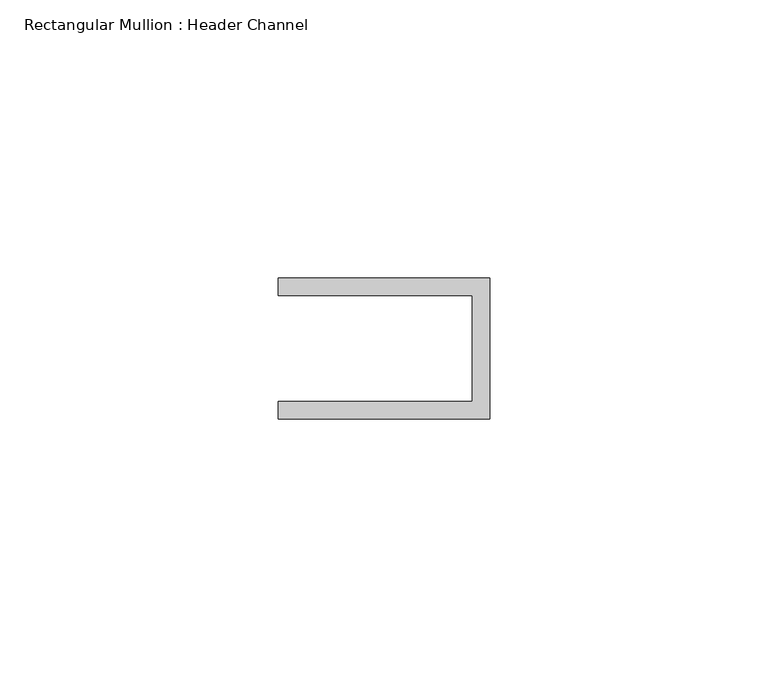
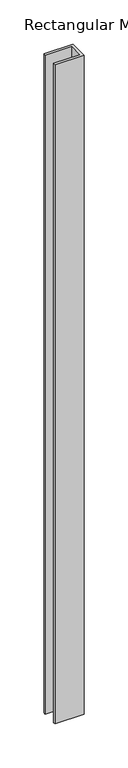
"""IFC4 building model written with IfcOpenShell, lengths in millimetres: member geometry, Rectangular Mullion : Header Channel."""

from ifc_helpers import new_model, si_unit, frame, origin, place, context, project, spatial, polyline, outline, extrude, source, transform, mapped, element, save


def rectangular_mullion_header_channel_2c3a6b86(model_context):
    return source(origin(), model_context, "Body", "SweptSolid", [
        extrude(outline(polyline([(0.0, -12.7), (-38.1, -12.7), (-38.1, -9.525), (-3.175, -9.525), (-3.175, 9.525), (-38.1, 9.525), (-38.1, 12.7), (0.0, 12.7), (0.0, -12.7)])), frame((0.0, 0.0, -914.4000002), z_axis=(0.0, 0.0, 1.0), x_axis=(1.0, 0.0, 0.0)), (0.0, 0.0, 1.0), 914.4000002),
    ])


if __name__ == "__main__":
    model = new_model("IFC4")
    model_context = context("Model", 3, world=origin())
    ifc_project = project(units=[si_unit("LENGTHUNIT", "METRE", prefix="MILLI")], contexts=[model_context])
    site = spatial("IfcSite", under=ifc_project)
    building = spatial("IfcBuilding", under=site)
    placement = place(None, origin())
    rectangular_mullion_header_channel_shape = rectangular_mullion_header_channel_2c3a6b86(model_context)
    element("IfcMember", 1, ObjectType="Rectangular Mullion : Header Channel", at=placement, inside=building, context=model_context, shape_type="MappedRepresentation", body=[
        mapped(rectangular_mullion_header_channel_shape, transform((0.0, 0.0, 0.0), x_axis=(1.0, 0.0, 0.0), y_axis=(0.0, 1.0, 0.0), z_axis=(0.0, 0.0, 1.0))),
    ])
    save(model, "model.ifc")

# Revit data of these elements
# Type "Rectangular Mullion : Header Channel"
#   built-in parameter 1007322 = 0.0833333 (stored number, unit not read)
#   built-in parameter 1007321 = -0.03125 (stored number, unit not read)
#   built-in parameter 1007320 = 0.0416667 (stored number, unit not read)
# Element 1 (IfcMember, "Rectangular Mullion : Header Channel")
#   Materials on its faces: "ALUM"
# Materials
#   "ALUM": class "Generic", colour RGB 157 157 157, transparency 0, Cost = 0
